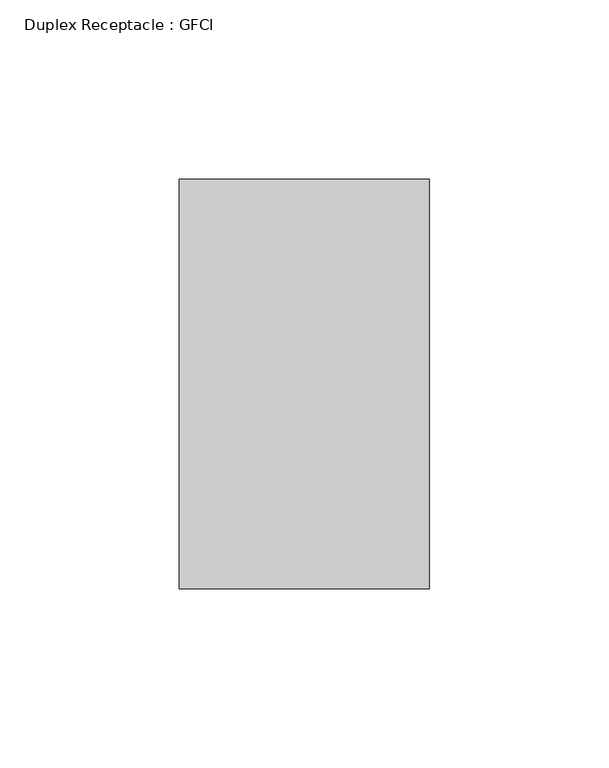
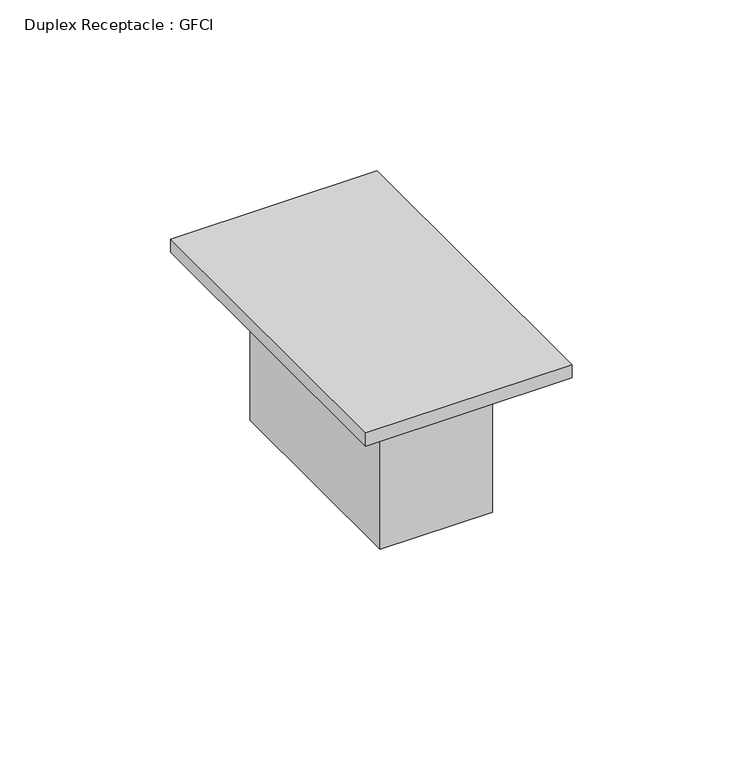
"""IFC4 building model written with IfcOpenShell, lengths in millimetres: proxy geometry, Duplex Receptacle : GFCI."""

from ifc_helpers import new_model, si_unit, frame, origin, origin_with_axes, place, context, project, spatial, polyline, outline, extrude, source, transform, mapped, element, save


def duplex_receptacle_gfci_88f187f2(model_context):
    return source(origin(), model_context, "Body", "SweptSolid", [
        extrude(outline(polyline([(19.05, -38.1), (-19.05, -38.1), (-19.05, 38.1), (19.05, 38.1), (19.05, -38.1)])), frame((0.0, 0.0, -53.975), z_axis=(0.0, 0.0, 1.0), x_axis=(1.0, 0.0, 0.0)), (0.0, 0.0, 1.0), 53.975),
        extrude(outline(polyline([(34.925, -57.15), (-34.925, -57.15), (-34.925, 57.15), (34.925, 57.15), (34.925, -57.15)])), origin_with_axes(), (0.0, 0.0, 1.0), 4.7625),
    ])


if __name__ == "__main__":
    model = new_model("IFC4")
    model_context = context("Model", 3, world=origin())
    ifc_project = project(units=[si_unit("LENGTHUNIT", "METRE", prefix="MILLI")], contexts=[model_context])
    site = spatial("IfcSite", under=ifc_project)
    building = spatial("IfcBuilding", under=site)
    placement = place(None, origin())
    duplex_receptacle_gfci_shape = duplex_receptacle_gfci_88f187f2(model_context)
    element("IfcBuildingElementProxy", 1, Name="Duplex Receptacle : GFCI", ObjectType="Duplex Receptacle : GFCI", at=placement, inside=building, context=model_context, shape_type="MappedRepresentation", body=[
        mapped(duplex_receptacle_gfci_shape, transform((0.0, 0.0, 0.0), x_axis=(1.0, 0.0, 0.0), y_axis=(0.0, 1.0, 0.0), z_axis=(0.0, 0.0, 1.0))),
    ])
    save(model, "model.ifc")

# Revit data of these elements
# Type "Duplex Receptacle : GFCI"
#   Label = "GFCI"
#   Switch Voltage = 120 V
#   Load = 180 VA
#   Default Elevation = 4' - 0"
#   Load Classification = Receptacle
#   Assembly Code = ""
